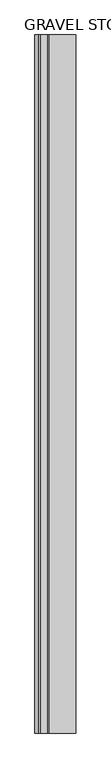
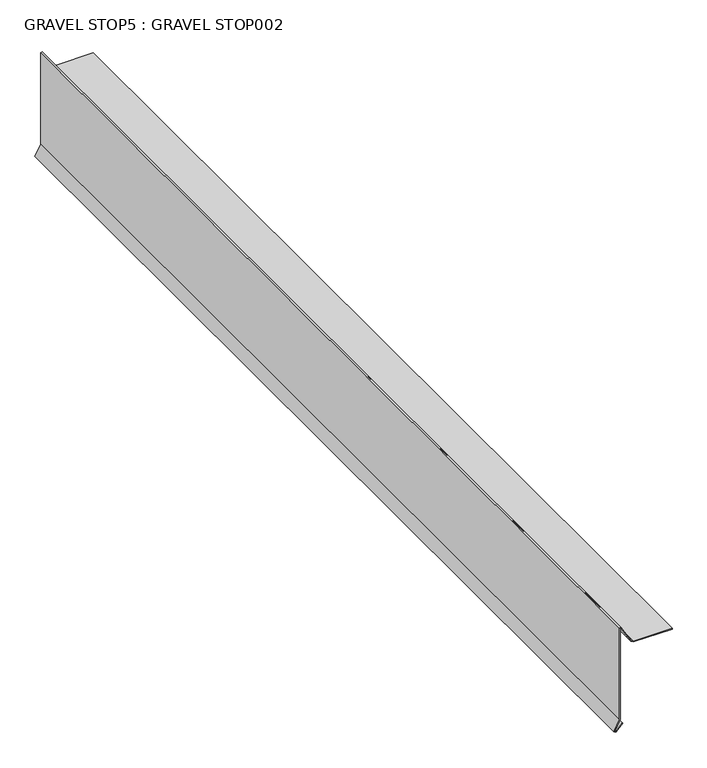
"""IFC4 building model written with IfcOpenShell, lengths in millimetres: proxy geometry, GRAVEL STOP5 : GRAVEL STOP002."""

from ifc_helpers import new_model, si_unit, frame, origin, place, context, project, spatial, polyline, outline, extrude, source, transform, mapped, element, save


def gravel_stop5_gravel_stop002_e62ea456(model_context):
    return source(origin(), model_context, "Body", "SweptSolid", [
        extrude(outline(polyline([(40077.410403, -5045.5157154), (40091.8049, -5031.1212184), (40092.8027062, -5032.1190245), (40079.2807815, -5045.6409492), (40080.9054201, -5047.7705993), (40101.495749, -5036.5295796), (40293.447969, -5036.5295796), (40293.699878, -5035.5894424), (40258.5078708, -5015.2713276), (40255.9633674, -5010.8641185), (40255.9633674, -4933.0281058), (40257.3744784, -4933.0281058), (40257.3744784, -5010.4860124), (40259.5408757, -5014.2383227), (40295.3431515, -5034.9087762), (40294.5307525, -5037.9406906), (40101.8558531, -5037.9406906), (40080.5182783, -5049.5896595), (40077.410403, -5045.5157154)])), frame((0.0, -1052.8906573, 0.0), z_axis=(0.0, 1.0, 0.0), x_axis=(0.0, 0.0, 1.0)), (0.0, 0.0, 1.0), 2000.25),
    ])


if __name__ == "__main__":
    model = new_model("IFC4")
    model_context = context("Model", 3, world=origin())
    ifc_project = project(units=[si_unit("LENGTHUNIT", "METRE", prefix="MILLI")], contexts=[model_context])
    site = spatial("IfcSite", under=ifc_project)
    building = spatial("IfcBuilding", under=site)
    placement = place(None, origin())
    gravel_stop5_gravel_stop002_shape = gravel_stop5_gravel_stop002_e62ea456(model_context)
    element("IfcBuildingElementProxy", 1, Name="GRAVEL STOP5 : GRAVEL STOP002", ObjectType="GRAVEL STOP5 : GRAVEL STOP002", at=placement, inside=building, context=model_context, shape_type="MappedRepresentation", body=[
        mapped(gravel_stop5_gravel_stop002_shape, transform((0.0, 0.0, 0.0), x_axis=(1.0, 0.0, 0.0), y_axis=(0.0, 1.0, 0.0), z_axis=(0.0, 0.0, 1.0))),
    ])
    save(model, "model.ifc")

# Revit data of these elements
# Type "GRAVEL STOP5 : GRAVEL STOP002"
#   NameOverride = "GRAVEL STOP002"
# Element 1 (IfcBuildingElementProxy, "GRAVEL STOP5 : GRAVEL STOP002")
#   Materials on its faces: "GRAVEL STOP REQUIRED WITH GRAVEL SURFACE SYSTEMS"
# Materials
#   "GRAVEL STOP REQUIRED WITH GRAVEL SURFACE SYSTEMS": class "Unassigned", colour RGB 170 170 127, transparency 0, Cost = 0
